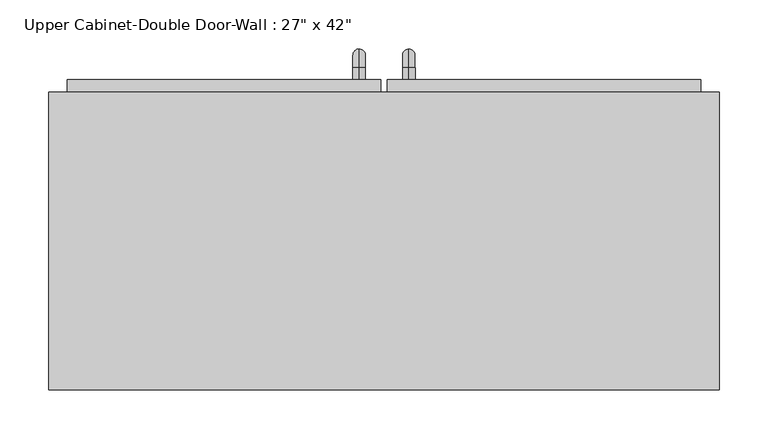
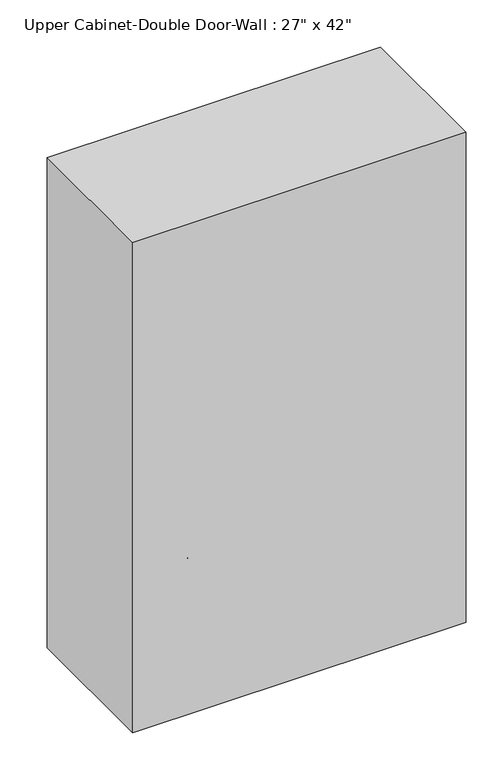
"""IFC4 building model written with IfcOpenShell, lengths in millimetres: furniture geometry."""

import ifcopenshell
import ifcopenshell.guid

model = None  # the IFC model being written
_history = None  # IfcOwnerHistory: only IFC2X3 demands one
_inside = {}  # id of a spatial element -> (the spatial element, [elements in it])
_under = {}  # id of a project, library or spatial element -> (it, [spatial elements below it])
_declared = {}  # id of a project -> (the project, [libraries it declares])
_typed = {}  # id of a type object -> (the type object, [elements of that type])
_made_of = {}  # id of a material, layer set ... -> (it, [elements and type objects made of it])


def new_model(schema):
    """Start an empty IFC model of exactly this schema.

    Asked for "IFC4X3", IfcOpenShell would pick the latest addendum, in which some entities
    have other attributes; the version numbers below select the first issue.
    IFC2X3 requires an IfcOwnerHistory on every rooted entity: one is made here for all.
    """
    global model, _history
    if schema == "IFC4X3":
        model = ifcopenshell.file(schema_version=(4, 3, 0, 0))
    else:
        model = ifcopenshell.file(schema=schema)
    _inside.clear()
    _under.clear()
    _declared.clear()
    _typed.clear()
    _made_of.clear()
    _history = None
    if model.schema == "IFC2X3":
        org = make("IfcOrganization", Name="unknown")
        user = make(
            "IfcPersonAndOrganization",
            ThePerson=make("IfcPerson", FamilyName="unknown"),
            TheOrganization=org,
        )
        app = make(
            "IfcApplication",
            ApplicationDeveloper=org,
            Version="unknown",
            ApplicationFullName="unknown",
            ApplicationIdentifier="unknown",
        )
        _history = make(
            "IfcOwnerHistory",
            OwningUser=user,
            OwningApplication=app,
            ChangeAction="ADDED",
            CreationDate=0,
        )
    return model


def make(cls, **values):
    """One entity of the class cls with the attributes given. An attribute that is None is left unset."""
    return model.create_entity(
        cls, **{name: value for name, value in values.items() if value is not None}
    )


def rooted(cls, **values):
    """An entity with a GlobalId (a new one), such as an element, a storey or a relation."""
    return make(cls, GlobalId=ifcopenshell.guid.new(), OwnerHistory=_history, **values)


def si_unit(unit_type, name, prefix=None):
    """IfcSIUnit, for example si_unit("LENGTHUNIT", "METRE", prefix="MILLI")."""
    return make("IfcSIUnit", UnitType=unit_type, Prefix=prefix, Name=name)


def assignment(units):
    """IfcUnitAssignment: the units of a project."""
    return None if units is None else make("IfcUnitAssignment", Units=units)


def point(xyz):
    """IfcCartesianPoint."""
    return None if xyz is None else make("IfcCartesianPoint", Coordinates=xyz)


def direction(xyz):
    """IfcDirection."""
    return None if xyz is None else make("IfcDirection", DirectionRatios=xyz)


def frame(location, z_axis=None, x_axis=None):
    """IfcAxis2Placement3D, a coordinate frame: its origin and axes. An axis left out is left unset."""
    return make(
        "IfcAxis2Placement3D",
        Location=point(location),
        Axis=direction(z_axis),
        RefDirection=direction(x_axis),
    )


def origin():
    """The frame at (0, 0, 0) with its axes left unset."""
    return frame((0.0, 0.0, 0.0))


def place(relative_to, where):
    """IfcLocalPlacement: puts the frame where relative to a parent placement (None: the world)."""
    return make(
        "IfcLocalPlacement", PlacementRelTo=relative_to, RelativePlacement=where
    )


def context(
    kind, dimensions, precision=None, world=None, true_north=None, identifier=None
):
    """IfcGeometricRepresentationContext, for example the 3D "Model" context."""
    return make(
        "IfcGeometricRepresentationContext",
        ContextIdentifier=identifier,
        ContextType=kind,
        CoordinateSpaceDimension=dimensions,
        Precision=precision,
        WorldCoordinateSystem=world,
        TrueNorth=true_north,
    )


def project(units=None, contexts=None):
    """IfcProject with its units and contexts."""
    return rooted(
        "IfcProject",
        Name="project",
        RepresentationContexts=contexts,
        UnitsInContext=assignment(units),
    )


def spatial(cls, under=None, at=None, **own):
    """A site, building, storey or space (cls), placed at a placement, below another one or the project."""
    s = rooted(cls, ObjectPlacement=at, **own)
    if under is not None:
        _under.setdefault(under.id(), (under, []))[1].append(s)
    return s


def polyline(points):
    """IfcPolyline through the points."""
    return make("IfcPolyline", Points=[point(p) for p in points])


def circle_curve(where, radius):
    """IfcCircle in the frame where."""
    return make("IfcCircle", Position=where, Radius=radius)


def ellipse_curve(where, semi_axis1, semi_axis2):
    """IfcEllipse in the frame where."""
    return make(
        "IfcEllipse", Position=where, SemiAxis1=semi_axis1, SemiAxis2=semi_axis2
    )


def trimmed(basis, trim1, trim2, sense, master):
    """IfcTrimmedCurve: the piece of a basis curve between two trims."""
    return make(
        "IfcTrimmedCurve",
        BasisCurve=basis,
        Trim1=trim1,
        Trim2=trim2,
        SenseAgreement=sense,
        MasterRepresentation=master,
    )


def outline(outer, holes=None, kind="AREA"):
    """IfcArbitraryClosedProfileDef: a profile drawn as a closed curve; with holes, ...WithVoids."""
    if holes is None:
        return make("IfcArbitraryClosedProfileDef", ProfileType=kind, OuterCurve=outer)
    return make(
        "IfcArbitraryProfileDefWithVoids",
        ProfileType=kind,
        OuterCurve=outer,
        InnerCurves=holes,
    )


def extrude(swept, where, along, depth):
    """IfcExtrudedAreaSolid: the profile swept, set in the frame where, extruded along a direction by depth."""
    return make(
        "IfcExtrudedAreaSolid",
        SweptArea=swept,
        Position=where,
        ExtrudedDirection=direction(along),
        Depth=depth,
    )


def faces_of(points, faces, orient=None, outer=None):
    """IfcFace entities. A face is a list of loops; a loop is a list of indices into points, from 0.

    orient and outer hold one flag for each loop. By default every Orientation is true, the
    first loop of a face is its IfcFaceOuterBound and the others are IfcFaceBound.
    """
    made = []
    for i, loops in enumerate(faces):
        bounds = []
        for j, loop in enumerate(loops):
            is_outer = j == 0 if outer is None else outer[i][j]
            bounds.append(
                make(
                    "IfcFaceOuterBound" if is_outer else "IfcFaceBound",
                    Bound=make("IfcPolyLoop", Polygon=[points[k] for k in loop]),
                    Orientation=True if orient is None else orient[i][j],
                )
            )
        made.append(make("IfcFace", Bounds=bounds))
    return made


def faceted_brep(points, faces, orient=None, outer=None, voids=None):
    """IfcFacetedBrep: a solid bounded by flat faces; with voids (closed shells), ...WithVoids."""
    shared = [point(p) for p in points]
    hull = make("IfcClosedShell", CfsFaces=faces_of(shared, faces, orient, outer))
    if voids is None:
        return make("IfcFacetedBrep", Outer=hull)
    return make(
        "IfcFacetedBrepWithVoids",
        Outer=hull,
        Voids=[
            make(cls, CfsFaces=faces_of(shared, fs, o, b)) for cls, fs, o, b in voids
        ],
    )


def shape(context_of_items, identifier, shape_type, items):
    """IfcShapeRepresentation: the items that make up one representation, for example the "Body"."""
    return make(
        "IfcShapeRepresentation",
        ContextOfItems=context_of_items,
        RepresentationIdentifier=identifier,
        RepresentationType=shape_type,
        Items=items,
    )


def source(mapping_origin, context_of_items, identifier, shape_type, items):
    """IfcRepresentationMap: a shape defined once, which mapped items show again and again."""
    return make(
        "IfcRepresentationMap",
        MappingOrigin=mapping_origin,
        MappedRepresentation=shape(context_of_items, identifier, shape_type, items),
    )


def transform(
    local_origin,
    x_axis=None,
    y_axis=None,
    z_axis=None,
    scale=None,
    scale2=None,
    scale3=None,
    uniform=True,
):
    """IfcCartesianTransformationOperator3D, or its non-uniform kind. x_axis, y_axis, z_axis: its Axis1, 2, 3."""
    if uniform:
        return make(
            "IfcCartesianTransformationOperator3D",
            Axis1=direction(x_axis),
            Axis2=direction(y_axis),
            LocalOrigin=point(local_origin),
            Scale=scale,
            Axis3=direction(z_axis),
        )
    return make(
        "IfcCartesianTransformationOperator3DnonUniform",
        Axis1=direction(x_axis),
        Axis2=direction(y_axis),
        LocalOrigin=point(local_origin),
        Scale=scale,
        Axis3=direction(z_axis),
        Scale2=scale2,
        Scale3=scale3,
    )


def mapped(mapping_source, mapping_target):
    """IfcMappedItem: shows the shape of a source again, moved by a transform."""
    return make(
        "IfcMappedItem", MappingSource=mapping_source, MappingTarget=mapping_target
    )


def made_of(thing, what):
    """Note that an element or type object is made of a material, layer set ...; save() writes the relation."""
    if what is not None:
        _made_of.setdefault(what.id(), (what, []))[1].append(thing)
    return thing


def element(
    cls,
    number,
    at=None,
    inside=None,
    cuts=None,
    type_object=None,
    material=None,
    context=None,
    identifier="Body",
    shape_type=None,
    held_by="IfcProductDefinitionShape",
    body=None,
    shapes=None,
    **own,
):
    """One element of the class cls, such as IfcWall. Its Tag is "e" and its number.

    at: its placement. inside: the storey or other place that contains it. cuts: it is an
    opening in that element (IfcRelVoidsElement). A single representation is given by context,
    identifier, shape_type and body (its items); several are given by shapes. held_by: the class
    of the entity that holds the representations. save() writes the other relations.
    """
    e = rooted(cls, Tag="e%d" % number, ObjectPlacement=at, **own)
    if body is not None:
        shapes = [shape(context, identifier, shape_type, body)]
    if shapes is not None:
        e.Representation = make(held_by, Representations=shapes)
    if inside is not None:
        _inside.setdefault(inside.id(), (inside, []))[1].append(e)
    if cuts is not None:
        rooted(
            "IfcRelVoidsElement", RelatingBuildingElement=cuts, RelatedOpeningElement=e
        )
    if type_object is not None:
        _typed.setdefault(type_object.id(), (type_object, []))[1].append(e)
    return made_of(e, material)


def aggregate(whole, parts):
    """IfcRelAggregates: a whole, such as a stair, and the parts it consists of."""
    return rooted("IfcRelAggregates", RelatingObject=whole, RelatedObjects=parts)


def save(model, path):
    """Write the relations noted so far, then the file.

    IfcRelAggregates (storeys below a building ...), IfcRelContainedInSpatialStructure (elements
    in a storey), IfcRelDefinesByType, IfcRelAssociatesMaterial and IfcRelDeclares: one each for
    every whole, place, type object, material and project.
    """
    for whole, parts in _under.values():
        aggregate(whole, parts)
    for where, things in _inside.values():
        rooted(
            "IfcRelContainedInSpatialStructure",
            RelatedElements=things,
            RelatingStructure=where,
        )
    for kind, things in _typed.values():
        rooted("IfcRelDefinesByType", RelatedObjects=things, RelatingType=kind)
    for what, things in _made_of.values():
        rooted("IfcRelAssociatesMaterial", RelatedObjects=things, RelatingMaterial=what)
    for by, libraries in _declared.values():
        rooted("IfcRelDeclares", RelatingContext=by, RelatedDefinitions=libraries)
    model.write(path)


def plane_surface(at):
    """IfcPlane: the flat surface through the origin of the frame at, square to its z axis."""
    return make("IfcPlane", Position=at)


def cylinder_surface(at, radius):
    """IfcCylindricalSurface: all points at the distance radius from the z axis of the frame at."""
    return make("IfcCylindricalSurface", Position=at, Radius=radius)


def revolved_surface(curve, axis_point, axis_direction):
    """IfcSurfaceOfRevolution: the curve turned about the line through axis_point along axis_direction."""
    return make(
        "IfcSurfaceOfRevolution",
        SweptCurve=make("IfcArbitraryOpenProfileDef", ProfileType="CURVE", Curve=curve),
        AxisPosition=make("IfcAxis1Placement", Location=point(axis_point), Axis=direction(axis_direction)),
    )


def advanced_brep(points, edges, surfaces, faces):
    """IfcAdvancedBrep: a solid bounded by faces that lie on surfaces and meet in shared edges.

    An edge is (start, end): straight between two places in points (the first is 0);
    or (start, end, curve); or (start, end, curve, False) where it runs against its curve.
    A face is (place in surfaces, loops), or (place, loops, False) where it looks against
    its surface's normal. A loop lists edges by number (the first is 1), with a minus sign
    where the edge is run from its end to its start. The first loop is the outer one.
    """
    corners = [point(p) for p in points]
    vertices = [make("IfcVertexPoint", VertexGeometry=c) for c in corners]
    made = []
    for start, end, *more in edges:
        made.append(
            make(
                "IfcEdgeCurve",
                EdgeStart=vertices[start],
                EdgeEnd=vertices[end],
                EdgeGeometry=more[0] if more else make("IfcPolyline", Points=[corners[start], corners[end]]),
                SameSense=more[1] if len(more) > 1 else True,
            )
        )
    hull = []
    for where, loops, *sense in faces:
        bounds = []
        for j, loop in enumerate(loops):
            ring = [make("IfcOrientedEdge", EdgeElement=made[abs(k) - 1], Orientation=k > 0) for k in loop]
            bounds.append(
                make(
                    "IfcFaceOuterBound" if j == 0 else "IfcFaceBound",
                    Bound=make("IfcEdgeLoop", EdgeList=ring),
                    Orientation=True,
                )
            )
        hull.append(make("IfcAdvancedFace", Bounds=bounds, FaceSurface=surfaces[where], SameSense=sense[0] if sense else True))
    return make("IfcAdvancedBrep", Outer=make("IfcClosedShell", CfsFaces=hull))


def furniture_9e6c3bdc(model_context):
    return source(origin(), model_context, "Body", "SolidModel", [
        faceted_brep([(-313.1288372, 80.9625, 2438.4), (-313.1288372, 80.9625, 1371.6), (372.6711628, 80.9625, 1371.6), (372.6711628, 80.9625, 2438.4), (-313.1288372, 385.7625, 2438.4), (372.6711628, 385.7625, 2438.4), (372.6711628, 385.7625, 1371.6), (-313.1288372, 385.7625, 1371.6), (-294.0788372, 385.7625, 2419.35), (-294.0788372, 385.7625, 1390.65), (353.6211628, 385.7625, 1390.65), (353.6211628, 385.7625, 2419.35), (353.6211628, 100.0125, 2419.35), (-294.0788372, 100.0125, 2419.35), (353.6211628, 100.0125, 1390.65), (-294.0788372, 100.0125, 1390.65)], [[[0, 1, 2, 3]], [[4, 5, 6, 7], [8, 9, 10, 11]], [[1, 0, 4, 7]], [[2, 1, 7, 6]], [[3, 2, 6, 5]], [[0, 3, 5, 4]], [[8, 11, 12, 13]], [[11, 10, 14, 12]], [[10, 9, 15, 14]], [[9, 8, 13, 15]], [[13, 12, 14, 15]]]),
        advanced_brep(
        [(55.1711628, 398.4625, 1517.65), (55.1711628, 398.4625, 1530.35), (55.1711628, 411.1625, 1517.65), (55.1711628, 411.1625, 1530.35), (55.1711628, 430.2125, 1511.3), (55.1711628, 417.5125, 1511.3), (55.1711628, 417.5125, 1435.1), (55.1711628, 430.2125, 1435.1), (55.1711628, 411.1625, 1416.05), (55.1711628, 411.1625, 1428.75), (55.1711628, 398.4625, 1428.75), (55.1711628, 398.4625, 1416.05)],
        [
            (0, 1, circle_curve(frame((55.1711628, 398.4625, 1524.0), z_axis=(0.0, -1.0, 0.0), x_axis=(0.0, 0.0, -1.0)), 6.35)),
            (1, 0, circle_curve(frame((55.1711628, 398.4625, 1524.0), z_axis=(0.0, -1.0, 0.0), x_axis=(0.0, 0.0, -1.0)), 6.35)),
            (0, 2),
            (2, 3, circle_curve(frame((55.1711628, 411.1625, 1524.0), z_axis=(0.0, -1.0, 0.0), x_axis=(0.0, 0.0, -1.0)), 6.35)),
            (3, 1),
            (3, 2, circle_curve(frame((55.1711628, 411.1625, 1524.0), z_axis=(0.0, -1.0, 0.0), x_axis=(0.0, 0.0, -1.0)), 6.35)),
            (4, 3, circle_curve(frame((55.1711628, 411.1625, 1511.3), z_axis=(1.0, 0.0, 0.0), x_axis=(0.0, 0.0, 1.0)), 19.05)),
            (2, 5, circle_curve(frame((55.1711628, 411.1625, 1511.3), z_axis=(-1.0, 0.0, 0.0), x_axis=(0.0, 0.0, 1.0)), 6.35)),
            (5, 4, circle_curve(frame((55.1711628, 423.8625, 1511.3), z_axis=(0.0, 0.0, 1.0), x_axis=(0.0, -1.0, 0.0)), 6.35)),
            (4, 5, circle_curve(frame((55.1711628, 423.8625, 1511.3), z_axis=(0.0, 0.0, 1.0), x_axis=(0.0, -1.0, 0.0)), 6.35)),
            (5, 6),
            (6, 7, circle_curve(frame((55.1711628, 423.8625, 1435.1), z_axis=(0.0, 0.0, 1.0), x_axis=(0.0, -1.0, 0.0)), 6.35)),
            (7, 4),
            (7, 6, circle_curve(frame((55.1711628, 423.8625, 1435.1), z_axis=(0.0, 0.0, 1.0), x_axis=(0.0, -1.0, 0.0)), 6.35)),
            (8, 7, circle_curve(frame((55.1711628, 411.1625, 1435.1), z_axis=(1.0, 0.0, 0.0), x_axis=(0.0, 1.0, 0.0)), 19.05)),
            (6, 9, circle_curve(frame((55.1711628, 411.1625, 1435.1), z_axis=(-1.0, 0.0, 0.0), x_axis=(0.0, 1.0, 0.0)), 6.35)),
            (9, 8, circle_curve(frame((55.1711628, 411.1625, 1422.4), z_axis=(0.0, 1.0, 0.0), x_axis=(0.0, 0.0, 1.0)), 6.35)),
            (8, 9, circle_curve(frame((55.1711628, 411.1625, 1422.4), z_axis=(0.0, 1.0, 0.0), x_axis=(0.0, 0.0, 1.0)), 6.35)),
            (10, 11, circle_curve(frame((55.1711628, 398.4625, 1422.4), z_axis=(0.0, -1.0, 0.0), x_axis=(0.0, 0.0, 1.0)), 6.35)),
            (11, 10, circle_curve(frame((55.1711628, 398.4625, 1422.4), z_axis=(0.0, -1.0, 0.0), x_axis=(0.0, 0.0, 1.0)), 6.35)),
            (9, 10),
            (11, 8),
        ],
        [
            plane_surface(frame((48.8211628, 398.4625, 1524.0), z_axis=(0.0, -1.0, 0.0), x_axis=(0.0, 0.0, 1.0))),
            cylinder_surface(frame((55.1711628, 398.4625, 1524.0), z_axis=(0.0, -1.0, 0.0), x_axis=(0.0, 0.0, -1.0)), 6.35),
            revolved_surface(trimmed(ellipse_curve(frame((55.1711628, 411.1625, 1524.0), z_axis=(0.0, -1.0, 0.0), x_axis=(0.0, 0.0, -1.0)), 6.35, 6.35), [point((55.1711628, 411.1625, 1517.65))], [point((55.1711628, 411.1625, 1530.35))], True, "CARTESIAN"), (55.1711628, 411.1625, 1511.3), (-1.0, 0.0, 0.0)),
            revolved_surface(trimmed(ellipse_curve(frame((55.1711628, 411.1625, 1524.0), z_axis=(0.0, -1.0, 0.0), x_axis=(0.0, 0.0, -1.0)), 6.35, 6.35), [point((55.1711628, 411.1625, 1530.35))], [point((55.1711628, 411.1625, 1517.65))], True, "CARTESIAN"), (55.1711628, 411.1625, 1511.3), (-1.0, 0.0, 0.0)),
            cylinder_surface(frame((55.1711628, 423.8625, 1511.3), z_axis=(0.0, 0.0, 1.0), x_axis=(0.0, -1.0, 0.0)), 6.35),
            revolved_surface(trimmed(ellipse_curve(frame((55.1711628, 423.8625, 1435.1), z_axis=(0.0, 0.0, 1.0), x_axis=(0.0, -1.0, 0.0)), 6.35, 6.35), [point((55.1711628, 417.5125, 1435.1))], [point((55.1711628, 430.2125, 1435.1))], True, "CARTESIAN"), (55.1711628, 411.1625, 1435.1), (-1.0, 0.0, 0.0)),
            revolved_surface(trimmed(ellipse_curve(frame((55.1711628, 423.8625, 1435.1), z_axis=(0.0, 0.0, 1.0), x_axis=(0.0, -1.0, 0.0)), 6.35, 6.35), [point((55.1711628, 430.2125, 1435.1))], [point((55.1711628, 417.5125, 1435.1))], True, "CARTESIAN"), (55.1711628, 411.1625, 1435.1), (-1.0, 0.0, 0.0)),
            plane_surface(frame((48.8211628, 398.4625, 1422.4), z_axis=(0.0, -1.0, 0.0), x_axis=(0.0, 0.0, -1.0))),
            cylinder_surface(frame((55.1711628, 411.1625, 1422.4), z_axis=(0.0, 1.0, 0.0), x_axis=(0.0, 0.0, 1.0)), 6.35),
        ],
        [
            (0, [[1, 2]]),
            (1, [[-1, 3, 4, 5]]),
            (1, [[-2, -5, 6, -3]]),
            (2, [[7, -4, 8, 9]]),
            (3, [[-8, -6, -7, 10]]),
            (4, [[-9, 11, 12, 13]]),
            (4, [[-10, -13, 14, -11]]),
            (5, [[15, -12, 16, 17]]),
            (6, [[-16, -14, -15, 18]]),
            (7, [[19, 20]]),
            (8, [[-17, 21, -20, 22]]),
            (8, [[-18, -22, -19, -21]]),
        ],
    ),
        advanced_brep(
        [(4.3711628, 398.4625, 1517.65), (4.3711628, 398.4625, 1530.35), (4.3711628, 411.1625, 1517.65), (4.3711628, 411.1625, 1530.35), (4.3711628, 430.2125, 1511.3), (4.3711628, 417.5125, 1511.3), (4.3711628, 417.5125, 1435.1), (4.3711628, 430.2125, 1435.1), (4.3711628, 411.1625, 1416.05), (4.3711628, 411.1625, 1428.75), (4.3711628, 398.4625, 1428.75), (4.3711628, 398.4625, 1416.05)],
        [
            (0, 1, circle_curve(frame((4.3711628, 398.4625, 1524.0), z_axis=(0.0, -1.0, 0.0), x_axis=(0.0, 0.0, 1.0)), 6.35)),
            (1, 0, circle_curve(frame((4.3711628, 398.4625, 1524.0), z_axis=(0.0, -1.0, 0.0), x_axis=(0.0, 0.0, 1.0)), 6.35)),
            (0, 2),
            (2, 3, circle_curve(frame((4.3711628, 411.1625, 1524.0), z_axis=(0.0, -1.0, 0.0), x_axis=(0.0, 0.0, 1.0)), 6.35)),
            (3, 1),
            (3, 2, circle_curve(frame((4.3711628, 411.1625, 1524.0), z_axis=(0.0, -1.0, 0.0), x_axis=(0.0, 0.0, 1.0)), 6.35)),
            (4, 3, circle_curve(frame((4.3711628, 411.1625, 1511.3), z_axis=(1.0, 0.0, 0.0), x_axis=(0.0, 0.0, 1.0)), 19.05)),
            (2, 5, circle_curve(frame((4.3711628, 411.1625, 1511.3), z_axis=(-1.0, 0.0, 0.0), x_axis=(0.0, 0.0, 1.0)), 6.35)),
            (5, 4, circle_curve(frame((4.3711628, 423.8625, 1511.3), z_axis=(0.0, 0.0, 1.0), x_axis=(0.0, 1.0, 0.0)), 6.35)),
            (4, 5, circle_curve(frame((4.3711628, 423.8625, 1511.3), z_axis=(0.0, 0.0, 1.0), x_axis=(0.0, 1.0, 0.0)), 6.35)),
            (5, 6),
            (6, 7, circle_curve(frame((4.3711628, 423.8625, 1435.1), z_axis=(0.0, 0.0, 1.0), x_axis=(0.0, 1.0, 0.0)), 6.35)),
            (7, 4),
            (7, 6, circle_curve(frame((4.3711628, 423.8625, 1435.1), z_axis=(0.0, 0.0, 1.0), x_axis=(0.0, 1.0, 0.0)), 6.35)),
            (8, 7, circle_curve(frame((4.3711628, 411.1625, 1435.1), z_axis=(1.0, 0.0, 0.0), x_axis=(0.0, 1.0, 0.0)), 19.05)),
            (6, 9, circle_curve(frame((4.3711628, 411.1625, 1435.1), z_axis=(-1.0, 0.0, 0.0), x_axis=(0.0, 1.0, 0.0)), 6.35)),
            (9, 8, circle_curve(frame((4.3711628, 411.1625, 1422.4), z_axis=(0.0, 1.0, 0.0), x_axis=(0.0, 0.0, -1.0)), 6.35)),
            (8, 9, circle_curve(frame((4.3711628, 411.1625, 1422.4), z_axis=(0.0, 1.0, 0.0), x_axis=(0.0, 0.0, -1.0)), 6.35)),
            (10, 11, circle_curve(frame((4.3711628, 398.4625, 1422.4), z_axis=(0.0, -1.0, 0.0), x_axis=(0.0, 0.0, -1.0)), 6.35)),
            (11, 10, circle_curve(frame((4.3711628, 398.4625, 1422.4), z_axis=(0.0, -1.0, 0.0), x_axis=(0.0, 0.0, -1.0)), 6.35)),
            (9, 10),
            (11, 8),
        ],
        [
            plane_surface(frame((-1.9788372, 398.4625, 1524.0), z_axis=(0.0, -1.0, 0.0), x_axis=(0.0, 0.0, 1.0))),
            cylinder_surface(frame((4.3711628, 398.4625, 1524.0), z_axis=(0.0, -1.0, 0.0), x_axis=(0.0, 0.0, 1.0)), 6.35),
            revolved_surface(trimmed(ellipse_curve(frame((4.3711628, 411.1625, 1524.0), z_axis=(0.0, -1.0, 0.0), x_axis=(0.0, 0.0, 1.0)), 6.35, 6.35), [point((4.3711628, 411.1625, 1517.65))], [point((4.3711628, 411.1625, 1530.35))], True, "CARTESIAN"), (4.3711628, 411.1625, 1511.3), (-1.0, 0.0, 0.0)),
            revolved_surface(trimmed(ellipse_curve(frame((4.3711628, 411.1625, 1524.0), z_axis=(0.0, -1.0, 0.0), x_axis=(0.0, 0.0, 1.0)), 6.35, 6.35), [point((4.3711628, 411.1625, 1530.35))], [point((4.3711628, 411.1625, 1517.65))], True, "CARTESIAN"), (4.3711628, 411.1625, 1511.3), (-1.0, 0.0, 0.0)),
            cylinder_surface(frame((4.3711628, 423.8625, 1511.3), z_axis=(0.0, 0.0, 1.0), x_axis=(0.0, 1.0, 0.0)), 6.35),
            revolved_surface(trimmed(ellipse_curve(frame((4.3711628, 423.8625, 1435.1), z_axis=(0.0, 0.0, 1.0), x_axis=(0.0, 1.0, 0.0)), 6.35, 6.35), [point((4.3711628, 417.5125, 1435.1))], [point((4.3711628, 430.2125, 1435.1))], True, "CARTESIAN"), (4.3711628, 411.1625, 1435.1), (-1.0, 0.0, 0.0)),
            revolved_surface(trimmed(ellipse_curve(frame((4.3711628, 423.8625, 1435.1), z_axis=(0.0, 0.0, 1.0), x_axis=(0.0, 1.0, 0.0)), 6.35, 6.35), [point((4.3711628, 430.2125, 1435.1))], [point((4.3711628, 417.5125, 1435.1))], True, "CARTESIAN"), (4.3711628, 411.1625, 1435.1), (-1.0, 0.0, 0.0)),
            plane_surface(frame((-1.9788372, 398.4625, 1422.4), z_axis=(0.0, -1.0, 0.0), x_axis=(0.0, 0.0, -1.0))),
            cylinder_surface(frame((4.3711628, 411.1625, 1422.4), z_axis=(0.0, 1.0, 0.0), x_axis=(0.0, 0.0, -1.0)), 6.35),
        ],
        [
            (0, [[1, 2]]),
            (1, [[-1, 3, 4, 5]]),
            (1, [[-2, -5, 6, -3]]),
            (2, [[7, -4, 8, 9]]),
            (3, [[-8, -6, -7, 10]]),
            (4, [[-9, 11, 12, 13]]),
            (4, [[-10, -13, 14, -11]]),
            (5, [[15, -12, 16, 17]]),
            (6, [[-16, -14, -15, 18]]),
            (7, [[19, 20]]),
            (8, [[-17, 21, -20, 22]]),
            (8, [[-18, -22, -19, -21]]),
        ],
    ),
        extrude(outline(polyline([(32.9461628, 398.4625), (353.6211628, 398.4625), (353.6211628, 366.7125), (32.9461628, 366.7125), (32.9461628, 398.4625)])), frame((0.0, 0.0, 1390.65), z_axis=(0.0, 0.0, 1.0), x_axis=(1.0, 0.0, 0.0)), (0.0, 0.0, 1.0), 1028.7),
        extrude(outline(polyline([(-294.0788372, 398.4625), (26.5961628, 398.4625), (26.5961628, 366.7125), (-294.0788372, 366.7125), (-294.0788372, 398.4625)])), frame((0.0, 0.0, 1390.65), z_axis=(0.0, 0.0, 1.0), x_axis=(1.0, 0.0, 0.0)), (0.0, 0.0, 1.0), 1028.7),
    ])


if __name__ == "__main__":
    model = new_model("IFC4")
    model_context = context("Model", 3, world=origin())
    ifc_project = project(units=[si_unit("LENGTHUNIT", "METRE", prefix="MILLI")], contexts=[model_context])
    site = spatial("IfcSite", under=ifc_project)
    building = spatial("IfcBuilding", under=site)
    placement = place(None, origin())
    furniture_shape = furniture_9e6c3bdc(model_context)
    element("IfcFurniture", 1, ObjectType="Upper Cabinet-Double Door-Wall : 27\" x 42\"", at=placement, inside=building, context=model_context, shape_type="MappedRepresentation", body=[
        mapped(furniture_shape, transform((0.0, 0.0, 0.0), x_axis=(1.0, 0.0, 0.0), y_axis=(0.0, 1.0, 0.0), z_axis=(0.0, 0.0, 1.0))),
    ])
    save(model, "model.ifc")

# Revit data of these elements
# Type "Upper Cabinet-Double Door-Wall : 27\" x 42\""
#   COBie.Type.CreatedBy = "doug.wood@us.ibm.com"
#   COBie.Type.CreatedOn = "2016-04-14T02:07:23"
#   COBie.Type.Name = "Casework_Upper Cabinet-Double Door-Wall_27\" x 42\""
#   COBie.Type.Category = "23-40 35 17 47 11 : Kitchen Casework"
#   COBie.Type.Description = "Upper Cabinet-Double Door-Wall_27\" x 42\""
#   COBie.Type.Manufacturer = ""
#   COBie.Type.ModelNumber = ""
#   Assembly Code = "C1030410"
#   COBie.Type.ReplacementCost = 0
#   Depth = 1' - 0"
#   Height = 3' - 6"
#   Top Of Cabinet = 8' - 0"
#   Width = 2' - 3"
#   COBie.Type = no
#   Cabinet Material = none
#   Door/Drawer Material = none
#   Handle Material = Cabinets - Handles
# Element 1 (IfcFurniture, "Upper Cabinet-Double Door-Wall : 27\" x 42\"")
#   Materials on its faces: "Cabinets - Handles", "Cabinets"
# Materials
#   "Cabinets - Handles": class "Metal", colour RGB 57 57 57, transparency 0
#   "Cabinets": class "Miscellaneous", colour RGB 249 249 249, transparency 0
